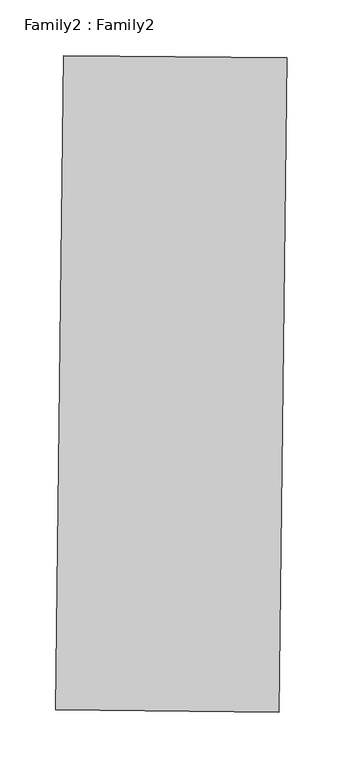
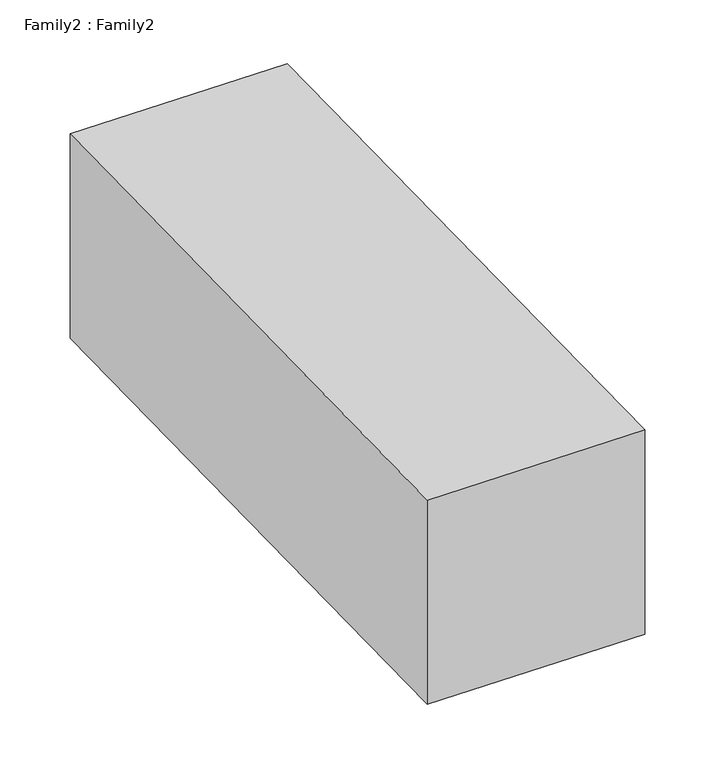
"""IFC4 building model written with IfcOpenShell, lengths in millimetres: proxy geometry, Family2 : Family2."""

from ifc_helpers import new_model, si_unit, origin, place, context, project, spatial, faceted_brep, source, transform, mapped, element, save


def family2_family2_6873a2fb(model_context):
    return source(origin(), model_context, "Body", "Brep", [
        faceted_brep([(-3946.9817223, -6366.3222661, 1.0945136), (-3946.9817223, -6366.3222661, 201.0945136), (-3939.8610722, -5781.2778565, 202.060409), (-3939.8610722, -5781.2778565, 2.060409), (-3746.9905323, -6368.1994787, 201.0945136), (-3739.8698823, -5783.1550692, 202.060409), (-3746.9905323, -6368.1994787, 1.0945136), (-3739.8698823, -5783.1550692, 2.060409)], [[[0, 1, 2, 3]], [[1, 4, 5, 2]], [[4, 6, 7, 5]], [[6, 0, 3, 7]], [[3, 2, 5, 7]], [[0, 6, 4, 1]]]),
    ])


if __name__ == "__main__":
    model = new_model("IFC4")
    model_context = context("Model", 3, world=origin())
    ifc_project = project(units=[si_unit("LENGTHUNIT", "METRE", prefix="MILLI")], contexts=[model_context])
    site = spatial("IfcSite", under=ifc_project)
    building = spatial("IfcBuilding", under=site)
    placement = place(None, origin())
    family2_family2_shape = family2_family2_6873a2fb(model_context)
    element("IfcBuildingElementProxy", 1, Name="Family2 : Family2", ObjectType="Family2 : Family2", at=placement, inside=building, context=model_context, shape_type="MappedRepresentation", body=[
        mapped(family2_family2_shape, transform((0.0, 0.0, 0.0), x_axis=(1.0, 0.0, 0.0), y_axis=(0.0, 1.0, 0.0), z_axis=(0.0, 0.0, 1.0))),
    ])
    save(model, "model.ifc")

# Revit data of these elements
# Type "Family2 : Family2"
#   Default Elevation = 0
